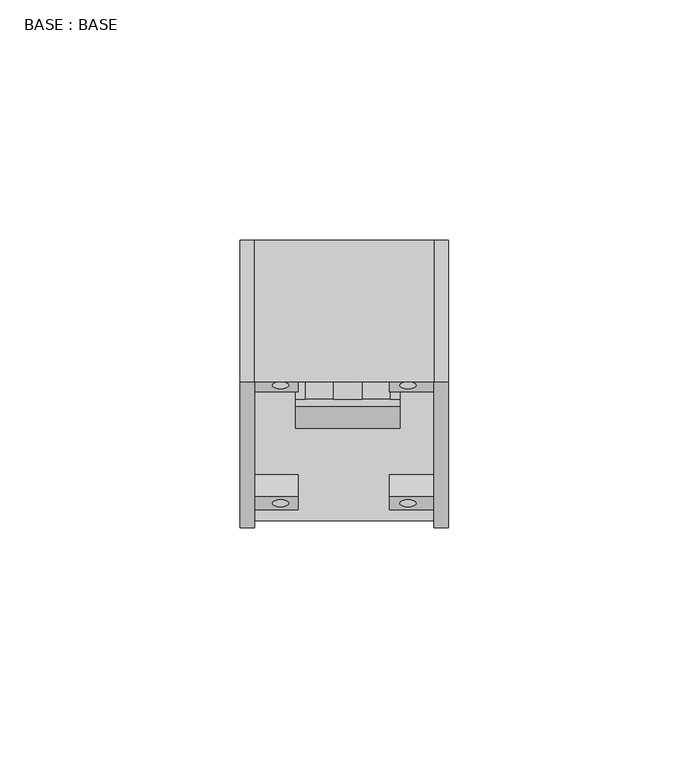
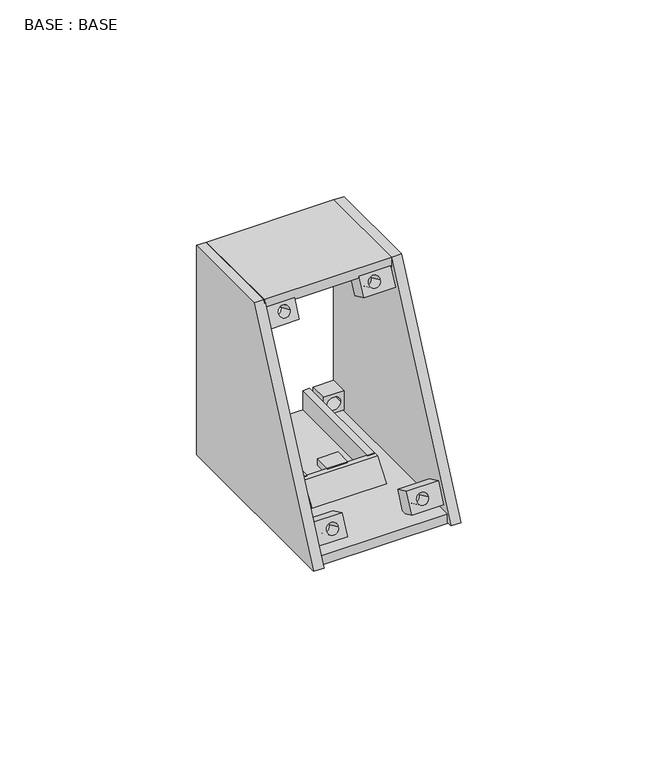
"""IFC4 building model written with IfcOpenShell, lengths in millimetres: proxy geometry, BASE : BASE."""

from ifc_helpers import new_model, si_unit, point, frame, frame_2d, origin, origin_with_axes, place, context, project, spatial, polyline, circle_curve, trimmed, segment, composite_curve, outline, extrude, source, transform, mapped, element, save


def base_base_600f8969(model_context):
    return source(origin(), model_context, "Body", "SweptSolid", [
        extrude(outline(polyline([(3.2, -2.2), (-3.2, -2.2), (-3.2, 7.1), (3.2, 7.1), (3.2, -2.2)]), holes=[composite_curve([segment(trimmed(circle_curve(frame_2d((0.0, 1.7)), 1.7), [point((0.0, 0.0))], [point((0.0, 3.4))], True, "CARTESIAN"), True, "CONTINUOUS"), segment(trimmed(circle_curve(frame_2d((0.0, 1.7)), 1.7), [point((0.0, 3.4))], [point((0.0, 0.0))], True, "CARTESIAN"), True, "CONTINUOUS")], self_intersect=False)]), frame((2402.2719295, 1326.1385366, 57.7208133), z_axis=(0.0, -0.9063077870366535, 0.4226182617406919), x_axis=(0.0, -0.4226182617406919, -0.9063077870366535)), (0.0, 0.0, 1.0), 5.0),
        extrude(outline(polyline([(3.2, -30.2), (-3.2, -30.2), (-3.2, -21.2), (3.2, -21.2), (3.2, -30.2)]), holes=[composite_curve([segment(trimmed(circle_curve(frame_2d((0.0, -24.8)), 1.7), [point((0.0, -23.1))], [point((0.0, -26.5))], True, "CARTESIAN"), True, "CONTINUOUS"), segment(trimmed(circle_curve(frame_2d((0.0, -24.8)), 1.7), [point((0.0, -26.5))], [point((0.0, -23.1))], True, "CARTESIAN"), True, "CONTINUOUS")], self_intersect=False)]), frame((2402.2719295, 1326.1385366, 57.7208133), z_axis=(0.0, -0.9063077870366535, 0.4226182617406919), x_axis=(0.0, -0.4226182617406919, -0.9063077870366535)), (0.0, 0.0, 1.0), 5.0),
        extrude(outline(polyline([(61.2, -2.2), (54.8, -2.2), (54.8, 7.1), (61.2, 7.1), (61.2, -2.2)]), holes=[composite_curve([segment(trimmed(circle_curve(frame_2d((58.0000001, 1.7)), 1.7), [point((58.0000001, 3.4))], [point((58.0000001, 0.0))], True, "CARTESIAN"), True, "CONTINUOUS"), segment(trimmed(circle_curve(frame_2d((58.0000001, 1.7)), 1.7), [point((58.0000001, 0.0))], [point((58.0000001, 3.4))], True, "CARTESIAN"), True, "CONTINUOUS")], self_intersect=False)]), frame((2402.2719295, 1326.1385366, 57.7208133), z_axis=(0.0, -0.9063077870366535, 0.4226182617406919), x_axis=(0.0, -0.4226182617406919, -0.9063077870366535)), (0.0, 0.0, 1.0), 5.0),
        extrude(outline(polyline([(61.2, -21.2), (61.2, -30.2), (54.8, -30.2), (54.8, -21.2), (61.2, -21.2)]), holes=[composite_curve([segment(trimmed(circle_curve(frame_2d((58.0000001, -24.8)), 1.7), [point((58.0000001, -23.1))], [point((58.0000001, -26.5))], True, "CARTESIAN"), True, "CONTINUOUS"), segment(trimmed(circle_curve(frame_2d((58.0000001, -24.8)), 1.7), [point((58.0000001, -26.5))], [point((58.0000001, -23.1))], True, "CARTESIAN"), True, "CONTINUOUS")], self_intersect=False)]), frame((2402.2719295, 1326.1385366, 57.7208133), z_axis=(0.0, -0.9063077870366535, 0.4226182617406919), x_axis=(0.0, -0.4226182617406919, -0.9063077870366535)), (0.0, 0.0, 1.0), 5.0),
        extrude(outline(polyline([(2394.4431854, 1318.7384159), (2388.4431854, 1318.7384159), (2388.4431854, 1323.7384159), (2394.4431854, 1323.7384159), (2394.4431854, 1318.7384159)])), frame((0.0, 0.0, 7.0), z_axis=(0.0, 0.0, 1.0), x_axis=(1.0, 0.0, 0.0)), (0.0, 0.0, 1.0), 2.0),
        extrude(outline(polyline([(1336.6555121, 3.0), (1344.7384159, 17.0), (1351.7384159, 17.0), (1351.7384159, 15.25), (1346.4884159, 15.25), (1346.4884159, 3.0), (1336.6555121, 3.0)])), frame((2372.0719295, 0.0, 0.0), z_axis=(1.0, 0.0, 0.0), x_axis=(0.0, 1.0, 0.0)), (0.0, 0.0, 1.0), 6.0),
        extrude(outline(polyline([(2409.3719295, 1322.3609206), (2372.0719295, 1322.3609206), (2372.0719295, 1351.7384159), (2409.3719295, 1351.7384159), (2409.3719295, 1322.3609206)])), frame((0.0, 0.0, 62.0), z_axis=(0.0, 0.0, 1.0), x_axis=(1.0, 0.0, 0.0)), (0.0, 0.0, 1.0), 3.0),
        extrude(outline(polyline([(3.0, 2403.3719295), (3.0, 2409.3719295), (9.0, 2409.3719295), (9.0, 2403.3719295), (3.0, 2403.3719295)]), holes=[composite_curve([segment(trimmed(circle_curve(frame_2d((6.0, 2406.3719295)), 2.0), [point((6.0, 2408.3719295))], [point((6.0, 2404.3719295))], True, "CARTESIAN"), True, "CONTINUOUS"), segment(trimmed(circle_curve(frame_2d((6.0, 2406.3719295)), 2.0), [point((6.0, 2404.3719295))], [point((6.0, 2408.3719295))], True, "CARTESIAN"), True, "CONTINUOUS")], self_intersect=False)]), frame((0.0, 1346.4884159, 0.0), z_axis=(0.0, 1.0, 0.0), x_axis=(0.0, 0.0, 1.0)), (0.0, 0.0, 1.0), 5.25),
        extrude(outline(polyline([(3.0, 2378.0719295), (9.0, 2378.0719295), (9.0, 2372.0719295), (3.0, 2372.0719295), (3.0, 2378.0719295)]), holes=[composite_curve([segment(trimmed(circle_curve(frame_2d((6.0, 2375.0719295)), 2.0), [point((6.0, 2377.0719295))], [point((6.0, 2373.0719295))], True, "CARTESIAN"), True, "CONTINUOUS"), segment(trimmed(circle_curve(frame_2d((6.0, 2375.0719295)), 2.0), [point((6.0, 2373.0719295))], [point((6.0, 2377.0719295))], True, "CARTESIAN"), True, "CONTINUOUS")], self_intersect=False)]), frame((0.0, 1346.4884159, 0.0), z_axis=(0.0, 1.0, 0.0), x_axis=(0.0, 0.0, 1.0)), (0.0, 0.0, 1.0), 5.25),
        extrude(outline(polyline([(62.0, 2403.3719295), (56.0, 2403.3719295), (56.0, 2409.3719295), (62.0, 2409.3719295), (62.0, 2403.3719295)]), holes=[composite_curve([segment(trimmed(circle_curve(frame_2d((59.0, 2406.3719295)), 2.0), [point((59.0, 2408.3719295))], [point((59.0, 2404.3719295))], True, "CARTESIAN"), True, "CONTINUOUS"), segment(trimmed(circle_curve(frame_2d((59.0, 2406.3719295)), 2.0), [point((59.0, 2404.3719295))], [point((59.0, 2408.3719295))], True, "CARTESIAN"), True, "CONTINUOUS")], self_intersect=False)]), frame((0.0, 1346.4884159, 0.0), z_axis=(0.0, 1.0, 0.0), x_axis=(0.0, 0.0, 1.0)), (0.0, 0.0, 1.0), 5.25),
        extrude(outline(polyline([(62.0, 2378.0719295), (62.0, 2372.0719295), (56.0, 2372.0719295), (56.0, 2378.0719295), (62.0, 2378.0719295)]), holes=[composite_curve([segment(trimmed(circle_curve(frame_2d((59.0, 2375.0719295)), 2.0), [point((59.0, 2377.0719295))], [point((59.0, 2373.0719295))], True, "CARTESIAN"), True, "CONTINUOUS"), segment(trimmed(circle_curve(frame_2d((59.0, 2375.0719295)), 2.0), [point((59.0, 2373.0719295))], [point((59.0, 2377.0719295))], True, "CARTESIAN"), True, "CONTINUOUS")], self_intersect=False)]), frame((0.0, 1346.4884159, 0.0), z_axis=(0.0, 1.0, 0.0), x_axis=(0.0, 0.0, 1.0)), (0.0, 0.0, 1.0), 5.25),
        extrude(outline(polyline([(1351.7384159, 0.0), (1292.0509228, 0.0), (1322.3609206, 65.0), (1351.7384159, 65.0), (1351.7384159, 0.0)])), frame((2409.3719295, 0.0, 0.0), z_axis=(1.0, 0.0, 0.0), x_axis=(0.0, 1.0, 0.0)), (0.0, 0.0, 1.0), 3.0),
        extrude(outline(polyline([(1351.7384159, 0.0), (1292.0509228, 0.0), (1322.3609206, 65.0), (1351.7384159, 65.0), (1351.7384159, 0.0)])), frame((2369.0719295, 0.0, 0.0), z_axis=(1.0, 0.0, 0.0), x_axis=(0.0, 1.0, 0.0)), (0.0, 0.0, 1.0), 3.0),
        extrude(outline(polyline([(2402.3331854, 1318.7384159), (2400.3331854, 1318.7384159), (2400.3331854, 1351.7384159), (2402.3331854, 1351.7384159), (2402.3331854, 1318.7384159)])), frame((0.0, 0.0, 3.0), z_axis=(0.0, 0.0, 1.0), x_axis=(1.0, 0.0, 0.0)), (0.0, 0.0, 1.0), 6.0),
        extrude(outline(polyline([(2380.5531854, 1318.7384159), (2380.5531854, 1351.7384159), (2382.5531854, 1351.7384159), (2382.5531854, 1318.7384159), (2380.5531854, 1318.7384159)])), frame((0.0, 0.0, 3.0), z_axis=(0.0, 0.0, 1.0), x_axis=(1.0, 0.0, 0.0)), (0.0, 0.0, 1.0), 6.0),
        extrude(outline(polyline([(1318.7384159, 9.0), (1318.7384159, 3.0), (1312.7384159, 3.0), (1317.2253325, 9.0), (1318.7384159, 9.0)])), frame((2380.5531854, 0.0, 0.0), z_axis=(1.0, 0.0, 0.0), x_axis=(0.0, 1.0, 0.0)), (0.0, 0.0, 1.0), 21.78),
        extrude(outline(polyline([(2409.3719295, 1293.4498458), (2372.0719295, 1293.4498458), (2372.0719295, 1351.7384159), (2409.3719295, 1351.7384159), (2409.3719295, 1293.4498458)])), origin_with_axes(), (0.0, 0.0, 1.0), 3.0),
    ])


if __name__ == "__main__":
    model = new_model("IFC4")
    model_context = context("Model", 3, world=origin())
    ifc_project = project(units=[si_unit("LENGTHUNIT", "METRE", prefix="MILLI")], contexts=[model_context])
    site = spatial("IfcSite", under=ifc_project)
    building = spatial("IfcBuilding", under=site)
    placement = place(None, origin())
    base_base_shape = base_base_600f8969(model_context)
    element("IfcBuildingElementProxy", 1, Name="BASE : BASE", ObjectType="BASE : BASE", at=placement, inside=building, context=model_context, shape_type="MappedRepresentation", body=[
        mapped(base_base_shape, transform((0.0, 0.0, 0.0), x_axis=(1.0, 0.0, 0.0), y_axis=(0.0, 1.0, 0.0), z_axis=(0.0, 0.0, 1.0))),
    ])
    save(model, "model.ifc")

# Revit data of these elements
# Element 1 (IfcBuildingElementProxy, "BASE : BASE")
#   Materials on its faces: ".BOX LATERAL"
# Materials
#   ".BOX LATERAL": class "Vidro", colour RGB 236 240 239, transparency 0.15, Cost = 0
